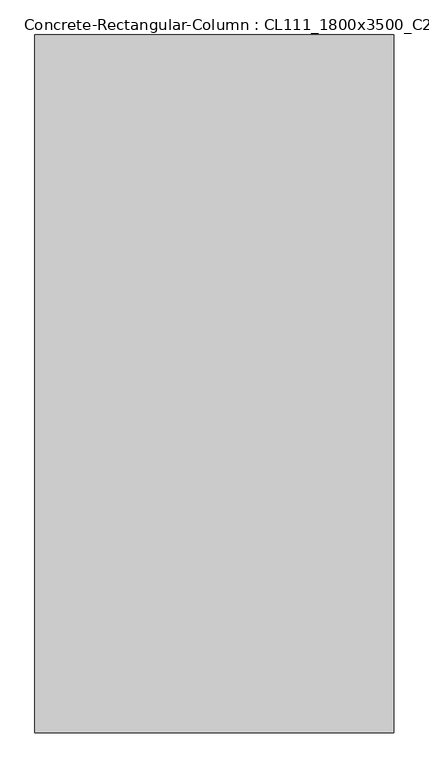
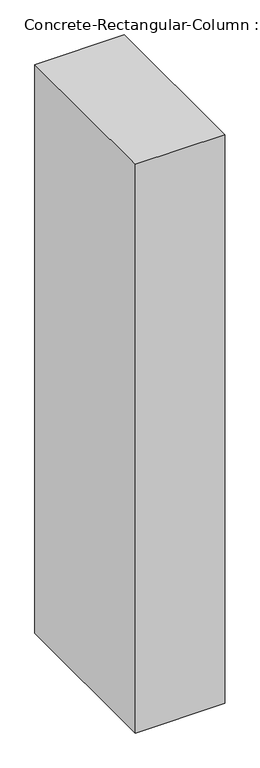
"""IFC4 building model written with IfcOpenShell, lengths in millimetres: column geometry, Concrete-Rectangular-Column : CL111_1800x3500_C2."""

from ifc_helpers import new_model, si_unit, frame, origin, place, context, project, spatial, polyline, outline, extrude, source, transform, mapped, element, save


def concrete_rectangular_column_cl111_1800x3500_c2_0d95458a(model_context):
    return source(origin(), model_context, "Body", "SweptSolid", [
        extrude(outline(polyline([(900.0, 1750.0), (900.0, -1750.0), (-900.0, -1750.0), (-900.0, 1750.0), (900.0, 1750.0)])), frame((0.0, 0.0, -2100.0), z_axis=(0.0, 0.0, 1.0), x_axis=(1.0, 0.0, 0.0)), (0.0, 0.0, 1.0), 12100.0),
    ])


if __name__ == "__main__":
    model = new_model("IFC4")
    model_context = context("Model", 3, world=origin())
    ifc_project = project(units=[si_unit("LENGTHUNIT", "METRE", prefix="MILLI")], contexts=[model_context])
    site = spatial("IfcSite", under=ifc_project)
    building = spatial("IfcBuilding", under=site)
    placement = place(None, origin())
    concrete_rectangular_column_cl111_1800x3500_c2_shape = concrete_rectangular_column_cl111_1800x3500_c2_0d95458a(model_context)
    element("IfcColumn", 1, ObjectType="Concrete-Rectangular-Column : CL111_1800x3500_C2", at=placement, inside=building, context=model_context, shape_type="MappedRepresentation", body=[
        mapped(concrete_rectangular_column_cl111_1800x3500_c2_shape, transform((0.0, 0.0, 0.0), x_axis=(1.0, 0.0, 0.0), y_axis=(0.0, 1.0, 0.0), z_axis=(0.0, 0.0, 1.0))),
    ])
    save(model, "model.ifc")

# Revit data of these elements
# Type "Concrete-Rectangular-Column : CL111_1800x3500_C2"
#   Description = "UG 철골 기둥용 Pedestal"
#   b = 1800 mm
#   h = 3500 mm
#   Width = 1800 mm
#   Length = 3500 mm
#   hec_material3 [instance default] = none
#   hec_material2 [instance default] = A03AE056-00001_Bitumen/Bituminous/Asphalt Coating
#   hec_material1 [instance default] = A03AC035-00001_Form Work (3 times in use)_Flat
#   Structural Material [instance default] = A03AC032-00007_Structural Concrete_Type1_25MPa-30Mpa
# Element 1 (IfcColumn, "Concrete-Rectangular-Column : CL111_1800x3500_C2")
#   hec_material2 = none
#   hec_material1 = none
#   Structural Material = 콘크리트 - 현장타설 콘크리트
#   Materials on its faces: "콘크리트 - 현장타설 콘크리트"
# Materials
#   "A03AE056-00001_Bitumen/Bituminous/Asphalt Coating": class "Generic", colour RGB 17 17 17, transparency 0, Description = "Damp-proofing", W00) Work Master Code = "A03AE056-00001", W01) Work Master_Lv1 = "Concrete Work", W02) Work Master_Lv2 = "Concrete Protective Coating (U/G)", W03) Work Master_Spec.1 = "Bitumen/Bituminous/Asphalt Coating", Cost = 0
#   "A03AC035-00001_Form Work (3 times in use)_Flat": class "Wood", colour RGB 149 120 74, transparency 0, Description = "Plywood", W00) Work Master Code = "A03AC035-00001", W01) Work Master_Lv1 = "Concrete Work", W02) Work Master_Lv2 = "Substructure Work", W03) Work Master_Spec.1 = "Form Work (3 times in use)", W04) Work Master_Spec.2 = "Flat Form", W05) Work Master_Spec.3 = "Dressed Lumber, Plywood or Steel Form(Wood Planks are not Allowed) incl. Chamfer", Cost = 0
#   "A03AC032-00007_Structural Concrete_Type1_25MPa-30Mpa": class "Concrete", colour RGB 176 176 176, transparency 0, Keynote = "09910.A1", Description = "Reinf. Conc.", W00) Work Master Code = "A03AC032-00007", W01) Work Master_Lv1 = "Concrete Work", W02) Work Master_Lv2 = "Substructure Work", W03) Work Master_Spec.1 = "Structural Concrete", W04) Work Master_Spec.2 = "Cement Type-1", W05) Work Master_Spec.3 = "25MPa < F'c (Cylinder Strength) ≤ 30MPa", Cost = 0
#   "콘크리트 - 현장타설 콘크리트": class "콘크리트", colour RGB 192 192 192, transparency 0
